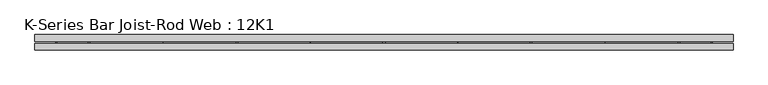
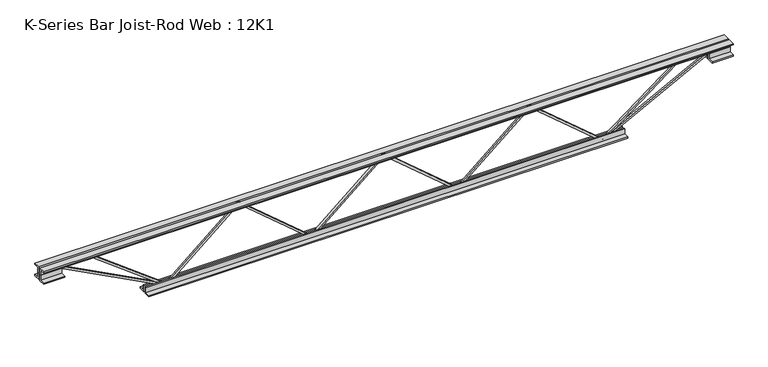
"""IFC4 building model written with IfcOpenShell, lengths in millimetres: beam geometry, K-Series Bar Joist-Rod Web : 12K1."""

import ifcopenshell
import ifcopenshell.guid

model = None  # the IFC model being written
_history = None  # IfcOwnerHistory: only IFC2X3 demands one
_inside = {}  # id of a spatial element -> (the spatial element, [elements in it])
_under = {}  # id of a project, library or spatial element -> (it, [spatial elements below it])
_declared = {}  # id of a project -> (the project, [libraries it declares])
_typed = {}  # id of a type object -> (the type object, [elements of that type])
_made_of = {}  # id of a material, layer set ... -> (it, [elements and type objects made of it])


def new_model(schema):
    """Start an empty IFC model of exactly this schema.

    Asked for "IFC4X3", IfcOpenShell would pick the latest addendum, in which some entities
    have other attributes; the version numbers below select the first issue.
    IFC2X3 requires an IfcOwnerHistory on every rooted entity: one is made here for all.
    """
    global model, _history
    if schema == "IFC4X3":
        model = ifcopenshell.file(schema_version=(4, 3, 0, 0))
    else:
        model = ifcopenshell.file(schema=schema)
    _inside.clear()
    _under.clear()
    _declared.clear()
    _typed.clear()
    _made_of.clear()
    _history = None
    if model.schema == "IFC2X3":
        org = make("IfcOrganization", Name="unknown")
        user = make(
            "IfcPersonAndOrganization",
            ThePerson=make("IfcPerson", FamilyName="unknown"),
            TheOrganization=org,
        )
        app = make(
            "IfcApplication",
            ApplicationDeveloper=org,
            Version="unknown",
            ApplicationFullName="unknown",
            ApplicationIdentifier="unknown",
        )
        _history = make(
            "IfcOwnerHistory",
            OwningUser=user,
            OwningApplication=app,
            ChangeAction="ADDED",
            CreationDate=0,
        )
    return model


def make(cls, **values):
    """One entity of the class cls with the attributes given. An attribute that is None is left unset."""
    return model.create_entity(
        cls, **{name: value for name, value in values.items() if value is not None}
    )


def rooted(cls, **values):
    """An entity with a GlobalId (a new one), such as an element, a storey or a relation."""
    return make(cls, GlobalId=ifcopenshell.guid.new(), OwnerHistory=_history, **values)


def si_unit(unit_type, name, prefix=None):
    """IfcSIUnit, for example si_unit("LENGTHUNIT", "METRE", prefix="MILLI")."""
    return make("IfcSIUnit", UnitType=unit_type, Prefix=prefix, Name=name)


def assignment(units):
    """IfcUnitAssignment: the units of a project."""
    return None if units is None else make("IfcUnitAssignment", Units=units)


def point(xyz):
    """IfcCartesianPoint."""
    return None if xyz is None else make("IfcCartesianPoint", Coordinates=xyz)


def direction(xyz):
    """IfcDirection."""
    return None if xyz is None else make("IfcDirection", DirectionRatios=xyz)


def frame(location, z_axis=None, x_axis=None):
    """IfcAxis2Placement3D, a coordinate frame: its origin and axes. An axis left out is left unset."""
    return make(
        "IfcAxis2Placement3D",
        Location=point(location),
        Axis=direction(z_axis),
        RefDirection=direction(x_axis),
    )


def origin():
    """The frame at (0, 0, 0) with its axes left unset."""
    return frame((0.0, 0.0, 0.0))


def place(relative_to, where):
    """IfcLocalPlacement: puts the frame where relative to a parent placement (None: the world)."""
    return make(
        "IfcLocalPlacement", PlacementRelTo=relative_to, RelativePlacement=where
    )


def context(
    kind, dimensions, precision=None, world=None, true_north=None, identifier=None
):
    """IfcGeometricRepresentationContext, for example the 3D "Model" context."""
    return make(
        "IfcGeometricRepresentationContext",
        ContextIdentifier=identifier,
        ContextType=kind,
        CoordinateSpaceDimension=dimensions,
        Precision=precision,
        WorldCoordinateSystem=world,
        TrueNorth=true_north,
    )


def project(units=None, contexts=None):
    """IfcProject with its units and contexts."""
    return rooted(
        "IfcProject",
        Name="project",
        RepresentationContexts=contexts,
        UnitsInContext=assignment(units),
    )


def spatial(cls, under=None, at=None, **own):
    """A site, building, storey or space (cls), placed at a placement, below another one or the project."""
    s = rooted(cls, ObjectPlacement=at, **own)
    if under is not None:
        _under.setdefault(under.id(), (under, []))[1].append(s)
    return s


def polyline(points):
    """IfcPolyline through the points."""
    return make("IfcPolyline", Points=[point(p) for p in points])


def outline(outer, holes=None, kind="AREA"):
    """IfcArbitraryClosedProfileDef: a profile drawn as a closed curve; with holes, ...WithVoids."""
    if holes is None:
        return make("IfcArbitraryClosedProfileDef", ProfileType=kind, OuterCurve=outer)
    return make(
        "IfcArbitraryProfileDefWithVoids",
        ProfileType=kind,
        OuterCurve=outer,
        InnerCurves=holes,
    )


def extrude(swept, where, along, depth):
    """IfcExtrudedAreaSolid: the profile swept, set in the frame where, extruded along a direction by depth."""
    return make(
        "IfcExtrudedAreaSolid",
        SweptArea=swept,
        Position=where,
        ExtrudedDirection=direction(along),
        Depth=depth,
    )


def shape(context_of_items, identifier, shape_type, items):
    """IfcShapeRepresentation: the items that make up one representation, for example the "Body"."""
    return make(
        "IfcShapeRepresentation",
        ContextOfItems=context_of_items,
        RepresentationIdentifier=identifier,
        RepresentationType=shape_type,
        Items=items,
    )


def source(mapping_origin, context_of_items, identifier, shape_type, items):
    """IfcRepresentationMap: a shape defined once, which mapped items show again and again."""
    return make(
        "IfcRepresentationMap",
        MappingOrigin=mapping_origin,
        MappedRepresentation=shape(context_of_items, identifier, shape_type, items),
    )


def transform(
    local_origin,
    x_axis=None,
    y_axis=None,
    z_axis=None,
    scale=None,
    scale2=None,
    scale3=None,
    uniform=True,
):
    """IfcCartesianTransformationOperator3D, or its non-uniform kind. x_axis, y_axis, z_axis: its Axis1, 2, 3."""
    if uniform:
        return make(
            "IfcCartesianTransformationOperator3D",
            Axis1=direction(x_axis),
            Axis2=direction(y_axis),
            LocalOrigin=point(local_origin),
            Scale=scale,
            Axis3=direction(z_axis),
        )
    return make(
        "IfcCartesianTransformationOperator3DnonUniform",
        Axis1=direction(x_axis),
        Axis2=direction(y_axis),
        LocalOrigin=point(local_origin),
        Scale=scale,
        Axis3=direction(z_axis),
        Scale2=scale2,
        Scale3=scale3,
    )


def mapped(mapping_source, mapping_target):
    """IfcMappedItem: shows the shape of a source again, moved by a transform."""
    return make(
        "IfcMappedItem", MappingSource=mapping_source, MappingTarget=mapping_target
    )


def made_of(thing, what):
    """Note that an element or type object is made of a material, layer set ...; save() writes the relation."""
    if what is not None:
        _made_of.setdefault(what.id(), (what, []))[1].append(thing)
    return thing


def element(
    cls,
    number,
    at=None,
    inside=None,
    cuts=None,
    type_object=None,
    material=None,
    context=None,
    identifier="Body",
    shape_type=None,
    held_by="IfcProductDefinitionShape",
    body=None,
    shapes=None,
    **own,
):
    """One element of the class cls, such as IfcWall. Its Tag is "e" and its number.

    at: its placement. inside: the storey or other place that contains it. cuts: it is an
    opening in that element (IfcRelVoidsElement). A single representation is given by context,
    identifier, shape_type and body (its items); several are given by shapes. held_by: the class
    of the entity that holds the representations. save() writes the other relations.
    """
    e = rooted(cls, Tag="e%d" % number, ObjectPlacement=at, **own)
    if body is not None:
        shapes = [shape(context, identifier, shape_type, body)]
    if shapes is not None:
        e.Representation = make(held_by, Representations=shapes)
    if inside is not None:
        _inside.setdefault(inside.id(), (inside, []))[1].append(e)
    if cuts is not None:
        rooted(
            "IfcRelVoidsElement", RelatingBuildingElement=cuts, RelatedOpeningElement=e
        )
    if type_object is not None:
        _typed.setdefault(type_object.id(), (type_object, []))[1].append(e)
    return made_of(e, material)


def aggregate(whole, parts):
    """IfcRelAggregates: a whole, such as a stair, and the parts it consists of."""
    return rooted("IfcRelAggregates", RelatingObject=whole, RelatedObjects=parts)


def save(model, path):
    """Write the relations noted so far, then the file.

    IfcRelAggregates (storeys below a building ...), IfcRelContainedInSpatialStructure (elements
    in a storey), IfcRelDefinesByType, IfcRelAssociatesMaterial and IfcRelDeclares: one each for
    every whole, place, type object, material and project.
    """
    for whole, parts in _under.values():
        aggregate(whole, parts)
    for where, things in _inside.values():
        rooted(
            "IfcRelContainedInSpatialStructure",
            RelatedElements=things,
            RelatingStructure=where,
        )
    for kind, things in _typed.values():
        rooted("IfcRelDefinesByType", RelatedObjects=things, RelatingType=kind)
    for what, things in _made_of.values():
        rooted("IfcRelAssociatesMaterial", RelatedObjects=things, RelatingMaterial=what)
    for by, libraries in _declared.values():
        rooted("IfcRelDeclares", RelatingContext=by, RelatedDefinitions=libraries)
    model.write(path)


def k_series_bar_joist_rod_web_12k1_aea474d1(model_context):
    return source(origin(), model_context, "Body", "SweptSolid", [
        extrude(outline(polyline([(-141.2875, -351.3666667), (-150.8125, -351.3666667), (-150.8125, -346.4463829), (141.2875, -1.4297162), (141.2875, 1.4297162), (-150.8125, 346.4463829), (-150.8125, 351.3666667), (-141.2875, 351.3666667), (-141.2875, 349.9369504), (150.8125, 4.9202838), (150.8125, -4.9202838), (-141.2875, -349.9369504), (-141.2875, -351.3666667)])), frame((0.0, -4.7625, 0.0), z_axis=(0.0, 1.0, 0.0), x_axis=(0.0, 0.0, 1.0)), (0.0, 0.0, 1.0), 9.525),
        extrude(outline(polyline([(-141.2875, 351.3666667), (-150.8125, 351.3666667), (-150.8125, 356.2869504), (141.2875, 701.3036171), (141.2875, 704.1630496), (-150.8125, 1049.1797162), (-150.8125, 1054.1), (-141.2875, 1054.1), (-141.2875, 1052.6702838), (150.8125, 707.6536171), (150.8125, 697.8130496), (-141.2875, 352.7963829), (-141.2875, 351.3666667)])), frame((0.0, -4.7625, 0.0), z_axis=(0.0, 1.0, 0.0), x_axis=(0.0, 0.0, 1.0)), (0.0, 0.0, 1.0), 9.525),
        extrude(outline(polyline([(-141.2875, -1054.1), (-150.8125, -1054.1), (-150.8125, -1049.1797162), (141.2875, -704.1630496), (141.2875, -701.3036171), (-150.8125, -356.2869504), (-150.8125, -351.3666667), (-141.2875, -351.3666667), (-141.2875, -352.7963829), (150.8125, -697.8130496), (150.8125, -707.6536171), (-141.2875, -1052.6702838), (-141.2875, -1054.1)])), frame((0.0, -4.7625, 0.0), z_axis=(0.0, 1.0, 0.0), x_axis=(0.0, 0.0, 1.0)), (0.0, 0.0, 1.0), 9.525),
        extrude(outline(polyline([(4.7625, 152.4), (36.5125, 152.4), (36.5125, 146.05), (11.1125, 146.05), (11.1125, 120.65), (4.7625, 120.65), (4.7625, 152.4)])), frame((-1663.7, 0.0, 0.0), z_axis=(1.0, 0.0, 0.0), x_axis=(0.0, 1.0, 0.0)), (0.0, 0.0, 1.0), 3327.4),
        extrude(outline(polyline([(-4.7625, 152.4), (-4.7625, 120.65), (-11.1125, 120.65), (-11.1125, 146.05), (-36.5125, 146.05), (-36.5125, 152.4), (-4.7625, 152.4)])), frame((-1663.7, 0.0, 0.0), z_axis=(1.0, 0.0, 0.0), x_axis=(0.0, 1.0, 0.0)), (0.0, 0.0, 1.0), 3327.4),
        extrude(outline(polyline([(-4.7625, 88.9), (-36.5125, 88.9), (-36.5125, 95.25), (-11.1125, 95.25), (-11.1125, 120.65), (-4.7625, 120.65), (-4.7625, 88.9)])), frame((-1663.7, 0.0, 0.0), z_axis=(1.0, 0.0, 0.0), x_axis=(0.0, 1.0, 0.0)), (0.0, 0.0, 1.0), 101.6),
        extrude(outline(polyline([(36.5125, 88.9), (4.7625, 88.9), (4.7625, 120.65), (11.1125, 120.65), (11.1125, 95.25), (36.5125, 95.25), (36.5125, 88.9)])), frame((-1663.7, 0.0, 0.0), z_axis=(1.0, 0.0, 0.0), x_axis=(0.0, 1.0, 0.0)), (0.0, 0.0, 1.0), 101.6),
        extrude(outline(polyline([(4.7625, 88.9), (4.7625, 120.65), (11.1125, 120.65), (11.1125, 95.25), (36.5125, 95.25), (36.5125, 88.9), (4.7625, 88.9)])), frame((1562.1, 0.0, 0.0), z_axis=(1.0, 0.0, 0.0), x_axis=(0.0, 1.0, 0.0)), (0.0, 0.0, 1.0), 101.6),
        extrude(outline(polyline([(-4.7625, 88.9), (-36.5125, 88.9), (-36.5125, 95.25), (-11.1125, 95.25), (-11.1125, 120.65), (-4.7625, 120.65), (-4.7625, 88.9)])), frame((1562.1, 0.0, 0.0), z_axis=(1.0, 0.0, 0.0), x_axis=(0.0, 1.0, 0.0)), (0.0, 0.0, 1.0), 101.6),
        extrude(outline(polyline([(4.7625, -152.4), (4.7625, -120.65), (11.1125, -120.65), (11.1125, -146.05), (36.5125, -146.05), (36.5125, -152.4), (4.7625, -152.4)])), frame((-1155.7, 0.0, 0.0), z_axis=(1.0, 0.0, 0.0), x_axis=(0.0, 1.0, 0.0)), (0.0, 0.0, 1.0), 2311.4),
        extrude(outline(polyline([(-4.7625, -152.4), (-36.5125, -152.4), (-36.5125, -146.05), (-11.1125, -146.05), (-11.1125, -120.65), (-4.7625, -120.65), (-4.7625, -152.4)])), frame((-1155.7, 0.0, 0.0), z_axis=(1.0, 0.0, 0.0), x_axis=(0.0, 1.0, 0.0)), (0.0, 0.0, 1.0), 2311.4),
        extrude(outline(polyline([(0.0, -9.525), (0.0, 0.0), (573.7533355, 0.0), (573.7533355, -9.525), (0.0, -9.525)])), frame((-1564.3137714, 4.7625, 116.4332925), z_axis=(0.46483389898951444, 0.0, 0.8853979028381567), x_axis=(0.8853979028381567, 0.0, -0.46483389898951444)), (0.0, 0.0, 1.0), 9.525),
        extrude(outline(polyline([(0.0, -9.525), (0.0, 0.0), (441.1206462, 0.0), (441.1206462, -9.525), (0.0, -9.525)])), frame((-1408.3460575, 4.7625, 116.8565168), z_axis=(0.6045965028797429, 0.0, 0.7965319006201729), x_axis=(0.7965319006201729, 0.0, -0.6045965028797429)), (0.0, 0.0, 1.0), 9.525),
        extrude(outline(polyline([(0.0, -9.525), (0.0, 0.0), (573.7533355, 0.0), (573.7533355, -9.525), (0.0, -9.525)])), frame((1564.3137714, -4.7625, 116.4332925), z_axis=(-0.4648338989894947, 0.0, 0.885397902838167), x_axis=(-0.885397902838167, 0.0, -0.4648338989894947)), (0.0, 0.0, 1.0), 9.525),
        extrude(outline(polyline([(0.0, -9.525), (0.0, 0.0), (441.1206462, 0.0), (441.1206462, -9.525), (0.0, -9.525)])), frame((1408.3460575, -4.7625, 116.8565168), z_axis=(-0.6045965028797365, 0.0, 0.7965319006201778), x_axis=(-0.7965319006201778, 0.0, -0.6045965028797365)), (0.0, 0.0, 1.0), 9.525),
    ])


if __name__ == "__main__":
    model = new_model("IFC4")
    model_context = context("Model", 3, world=origin())
    ifc_project = project(units=[si_unit("LENGTHUNIT", "METRE", prefix="MILLI")], contexts=[model_context])
    site = spatial("IfcSite", under=ifc_project)
    building = spatial("IfcBuilding", under=site)
    placement = place(None, origin())
    k_series_bar_joist_rod_web_12k1_shape = k_series_bar_joist_rod_web_12k1_aea474d1(model_context)
    element("IfcBeam", 1, ObjectType="K-Series Bar Joist-Rod Web : 12K1", at=placement, inside=building, context=model_context, shape_type="MappedRepresentation", body=[
        mapped(k_series_bar_joist_rod_web_12k1_shape, transform((0.0, 0.0, 0.0), x_axis=(1.0, 0.0, 0.0), y_axis=(0.0, 1.0, 0.0), z_axis=(0.0, 0.0, 1.0))),
    ])
    save(model, "model.ifc")

# Revit data of these elements
# Type "K-Series Bar Joist-Rod Web : 12K1"
#   Assembly Code = "B1010350"
#   Wt = 5
#   Web Thickness = 0' - 0 3/8"
#   Start Offset [instance default] = 0' - 0"
#   Start Extension [instance default] = 0' - 0"
#   Seat Length = 0' - 4"
#   Seat Depth = 0' - 2 1/2"
#   PanelArrayLength [instance default] = 20' - 0"
#   Panel [instance default] = 2' - 0"
#   End Offset [instance default] = 0' - 0"
#   End Extension [instance default] = 0' - 0"
#   End Panel = 2' - 0"
#   Cord Leg = 0' - 1 1/4"
#   Chord Thickness = 0' - 0 1/4"
#   Length [instance default] = 24' - 0"
#   Depth = 1' - 0"
#   PanelArrayNum [instance default] = 10
#   Structural Material = none
# Element 1 (IfcBeam, "K-Series Bar Joist-Rod Web : 12K1")
#   PanelArrayLength = 6' - 11"
#   Panel = 2' - 3.66667"
#   PanelArrayNum = 3
